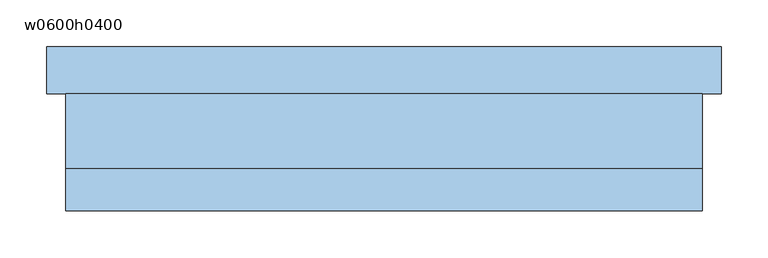
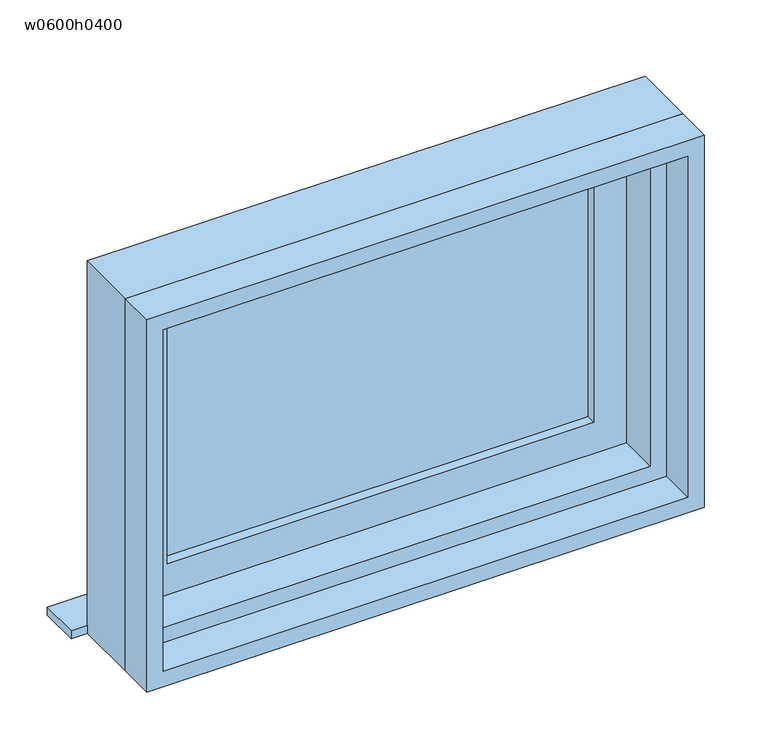
"""IFC4 building model written with IfcOpenShell, lengths in millimetres: window geometry, 横すべり窓 : w0600h0400."""

from ifc_helpers import new_model, si_unit, frame, origin, place, context, project, spatial, polyline, outline, extrude, source, transform, mapped, element, save


def w0600h0400_4ba1228e(model_context):
    return source(origin(), model_context, "Body", "SweptSolid", [
        extrude(outline(polyline([(260.0, 22.5), (-260.0, 22.5), (-260.0, 27.5), (260.0, 27.5), (260.0, 22.5)])), frame((0.0, 0.0, 1640.0), z_axis=(0.0, 0.0, 1.0), x_axis=(1.0, 0.0, 0.0)), (0.0, 0.0, 1.0), 320.0),
        extrude(outline(polyline([(2000.0, 300.0), (2000.0, -300.0), (1600.0, -300.0), (1600.0, 300.0), (2000.0, 300.0)]), holes=[polyline([(1960.0, -260.0), (1960.0, 260.0), (1640.0, 260.0), (1640.0, -260.0), (1960.0, -260.0)])]), frame((0.0, 10.0, 0.0), z_axis=(0.0, 1.0, 0.0), x_axis=(0.0, 0.0, 1.0)), (0.0, 0.0, 1.0), 30.0),
        extrude(outline(polyline([(360.0, 90.0), (360.0, 40.0), (-360.0, 40.0), (-360.0, 90.0), (360.0, 90.0)])), frame((0.0, 0.0, 1560.0), z_axis=(0.0, 0.0, 1.0), x_axis=(1.0, 0.0, 0.0)), (0.0, 0.0, 1.0), 10.0),
        extrude(outline(polyline([(2040.0, 340.0), (2040.0, -340.0), (1560.0, -340.0), (1560.0, 340.0), (2040.0, 340.0)]), holes=[polyline([(1580.0, -320.0), (2020.0, -320.0), (2020.0, 320.0), (1580.0, 320.0), (1580.0, -320.0)])]), frame((0.0, -85.0, 0.0), z_axis=(0.0, 1.0, 0.0), x_axis=(0.0, 0.0, 1.0)), (0.0, 0.0, 1.0), 45.0),
        extrude(outline(polyline([(2040.0, -340.0), (1560.0, -340.0), (1560.0, 340.0), (2040.0, 340.0), (2040.0, -340.0)]), holes=[polyline([(2000.0, 300.0), (1600.0, 300.0), (1600.0, -300.0), (2000.0, -300.0), (2000.0, 300.0)])]), frame((0.0, -40.0, 0.0), z_axis=(0.0, 1.0, 0.0), x_axis=(0.0, 0.0, 1.0)), (0.0, 0.0, 1.0), 80.0),
    ])


if __name__ == "__main__":
    model = new_model("IFC4")
    model_context = context("Model", 3, world=origin())
    ifc_project = project(units=[si_unit("LENGTHUNIT", "METRE", prefix="MILLI")], contexts=[model_context])
    site = spatial("IfcSite", under=ifc_project)
    building = spatial("IfcBuilding", under=site)
    placement = place(None, origin())
    w0600h0400_shape = w0600h0400_4ba1228e(model_context)
    element("IfcWindow", 1, ObjectType="横すべり窓 : w0600h0400", at=placement, inside=building, context=model_context, shape_type="MappedRepresentation", body=[
        mapped(w0600h0400_shape, transform((0.0, 0.0, 0.0), x_axis=(1.0, 0.0, 0.0), y_axis=(0.0, 1.0, 0.0), z_axis=(0.0, 0.0, 1.0))),
    ])
    save(model, "model.ifc")

# Revit data of these elements
# Type "横すべり窓 : w0600h0400"
#   Construction Type Id = "GSP4R"
#   Analytic Construction = "1/8 インチ ピルキントン一重ガラス"
#   Type Mark = "76"
#   Operation = "シングルパネル"
#   Keynote = "08520.S1"
#   Visual Light Transmittance = 0.9
#   Solar Heat Gain Coefficient = 0.86
#   Heat Transfer Coefficient (U) = 6.7069 W/(m²·K)
#   Height = 400 mm
#   既定の腰高 = 1600 mm
#   Width = 600 mm
#   額縁見附 = 20 mm
#   額縁ちり = 10 mm
#   サッシ見附 = 40 mm
#   サッシの幅 = 80 mm
#   サッシ額縁 [instance default] = none
#   サッシ本体 [instance default] = none
#   サッシガラス [instance default] = ガラス - 透明
#   Wall Closure = (empty or 0)
#   Type Comments = ""
#   Assembly Code = ""
# Element 1 (IfcWindow, "横すべり窓 : w0600h0400")
#   Materials on its faces: "ガラス - 透明"
# Materials
#   "ガラス - 透明": class "ガラス", colour RGB 0 128 192, transparency 0.9, Cost = 0
